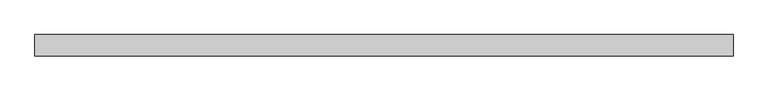
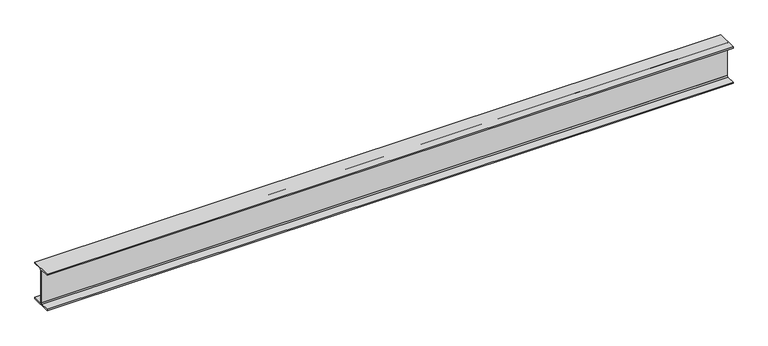
"""IFC4 building model written with IfcOpenShell, lengths in millimetres: beam geometry, Old_Steel Beam_H-KSD3502 : H_SB_ASB_H-200×200x8x12."""

from ifc_helpers import new_model, si_unit, point, frame, frame_2d, origin, place, context, project, spatial, polyline, circle_curve, trimmed, segment, composite_curve, outline, extrude, source, transform, mapped, element, save


def beam_d25946cc(model_context):
    return source(origin(), model_context, "Body", "SweptSolid", [
        extrude(outline(composite_curve([segment(polyline([(82.5, -141.5), (82.5, -151.7), (-82.5, -151.7), (-82.5, -141.5), (-11.9, -141.5)]), True, "CONTINUOUS"), segment(trimmed(circle_curve(frame_2d((-11.9, -132.6)), 8.9), [point((-11.9, -141.5))], [point((-3.0, -132.6))], True, "CARTESIAN"), True, "CONTINUOUS"), segment(polyline([(-3.0, -132.6), (-3.0, 132.6)]), True, "CONTINUOUS"), segment(trimmed(circle_curve(frame_2d((-11.9, 132.6)), 8.9), [point((-3.0, 132.6))], [point((-11.9, 141.5))], True, "CARTESIAN"), True, "CONTINUOUS"), segment(polyline([(-11.9, 141.5), (-82.5, 141.5), (-82.5, 151.7), (82.5, 151.7), (82.5, 141.5), (11.9, 141.5)]), True, "CONTINUOUS"), segment(trimmed(circle_curve(frame_2d((11.9, 132.6)), 8.9), [point((11.9, 141.5))], [point((3.0, 132.6))], True, "CARTESIAN"), True, "CONTINUOUS"), segment(polyline([(3.0, 132.6), (3.0, -132.6)]), True, "CONTINUOUS"), segment(trimmed(circle_curve(frame_2d((11.9, -132.6)), 8.9), [point((3.0, -132.6))], [point((11.9, -141.5))], True, "CARTESIAN"), True, "CONTINUOUS"), segment(polyline([(11.9, -141.5), (82.5, -141.5)]), True, "CONTINUOUS")], self_intersect=False)), frame((-2711.6798, 0.0, 0.0), z_axis=(1.0, 0.0, 0.0), x_axis=(0.0, 1.0, 0.0)), (0.0, 0.0, 1.0), 5395.0201602),
    ])


if __name__ == "__main__":
    model = new_model("IFC4")
    model_context = context("Model", 3, world=origin())
    ifc_project = project(units=[si_unit("LENGTHUNIT", "METRE", prefix="MILLI")], contexts=[model_context])
    site = spatial("IfcSite", under=ifc_project)
    building = spatial("IfcBuilding", under=site)
    placement = place(None, origin())
    beam_shape = beam_d25946cc(model_context)
    element("IfcBeam", 1, ObjectType="Old_Steel Beam_H-KSD3502 : H_SB_ASB_H-200×200x8x12", at=placement, inside=building, context=model_context, shape_type="MappedRepresentation", body=[
        mapped(beam_shape, transform((0.0, 0.0, 0.0), x_axis=(1.0, 0.0, 0.0), y_axis=(0.0, 1.0, 0.0), z_axis=(0.0, 0.0, 1.0))),
    ])
    save(model, "model.ifc")

# Revit data of these elements
# Type "Old_Steel Beam_H-KSD3502 : H_SB_ASB_H-200×200x8x12"
#   Width = 20.0 cm
#   Web Thickness = 0.8 cm
#   Web Fillet = 1.3 cm
#   Warping Constant = 141376.0 cm⁶
#   Torsional Moment of Inertia = 26.2485 cm⁴
#   Torsional Modulus = 1.0 cm³
#   Section Area = 63.53 cm²
#   Plastic Modulus weak axis = 244.0 cm³
#   Plastic Modulus strong axis = 525.0 cm³
#   Perimeter = 1.16 m²/m
#   Nominal Weight = 49.90 kgf/m
#   Moment of Inertia weak axis = 1600.00 cm⁴
#   Moment of Inertia strong axis = 4720.00 cm⁴
#   Height = 20.0 cm
#   Flange Thickness = 1.2 cm
#   Elastic Modulus weak axis = 160.0 cm³
#   Elastic Modulus strong axis = 472.0 cm³
#   Centroid Vertical = 10.0 cm
#   Centroid Horizontal = 10.0 cm
#   Length [instance default] = 1.5240 m
#   Structural Material [instance default] = Steel, 45-345
#   Assembly Code = ""
# Element 1 (IfcBeam, "Old_Steel Beam_H-KSD3502 : H_SB_ASB_H-200×200x8x12")
#   Structural Material = none
# Materials
#   "Steel, 45-345": class "Metal", colour RGB 189 187 185, transparency 0, Description = "Steel 345 MPa", Cost = 0
